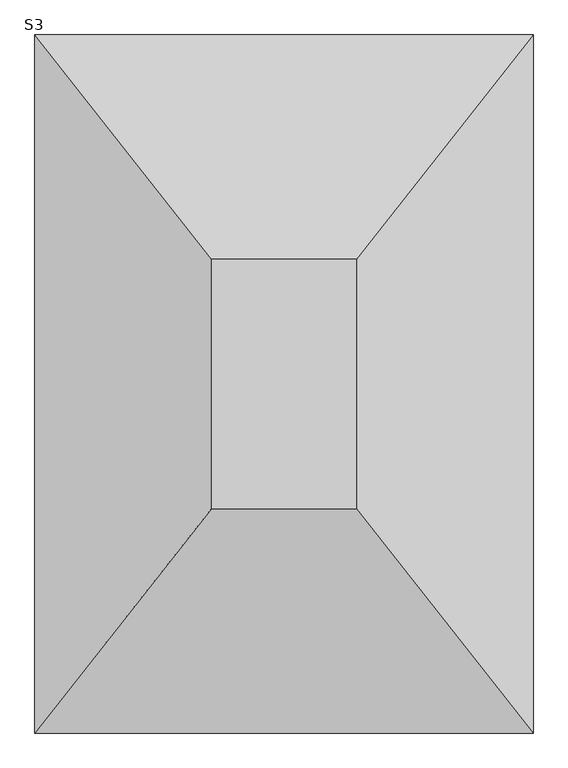
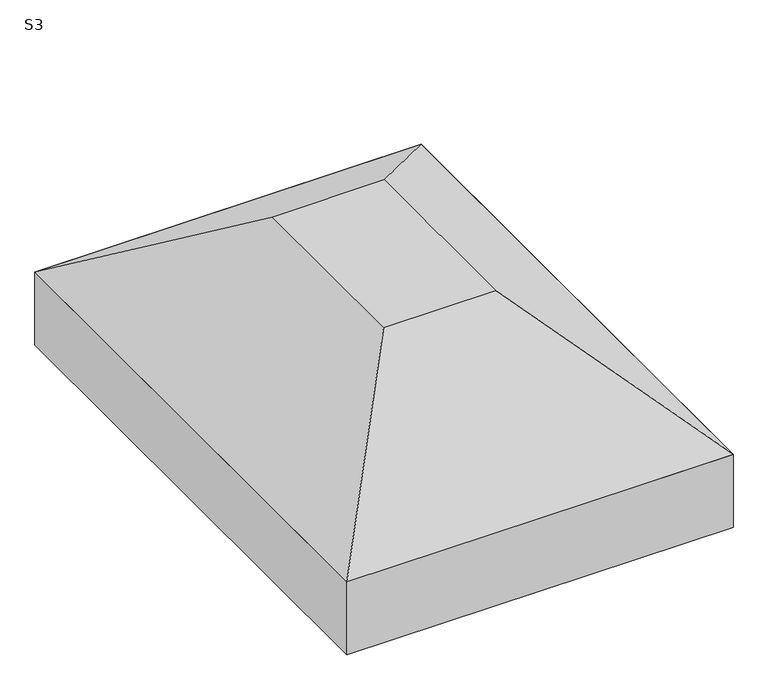
"""IFC4 building model written with IfcOpenShell, lengths in millimetres: fastener geometry, TQS - Sapata : S3."""

from ifc_helpers import new_model, si_unit, frame, origin, place, context, project, spatial, polyline, outline, extrude, faceted_brep, source, transform, mapped, element, save


def s3_fc183e28(model_context):
    return source(origin(), model_context, "Body", "SolidModel", [
        faceted_brep([(-55.0, 50.0, 0.0), (-345.0, 50.0, 0.0), (-345.0, -450.0, 0.0), (-55.0, -450.0, 0.0), (300.0, 500.0, -300.0), (300.0, -900.0, -300.0), (-700.0, -900.0, -300.0), (-700.0, 500.0, -300.0)], [[[0, 1, 2, 3]], [[4, 5, 6, 7]], [[4, 7, 1, 0]], [[7, 6, 2, 1]], [[6, 5, 3, 2]], [[5, 4, 0, 3]]]),
        extrude(outline(polyline([(300.0, 500.0), (300.0, -900.0), (-700.0, -900.0), (-700.0, 500.0), (300.0, 500.0)])), frame((0.0, 0.0, -500.0), z_axis=(0.0, 0.0, 1.0), x_axis=(1.0, 0.0, 0.0)), (0.0, 0.0, 1.0), 200.0),
    ])


if __name__ == "__main__":
    model = new_model("IFC4")
    model_context = context("Model", 3, world=origin())
    ifc_project = project(units=[si_unit("LENGTHUNIT", "METRE", prefix="MILLI")], contexts=[model_context])
    site = spatial("IfcSite", under=ifc_project)
    building = spatial("IfcBuilding", under=site)
    placement = place(None, origin())
    s3_shape = s3_fc183e28(model_context)
    element("IfcFastener", 1, ObjectType="TQS - Sapata : S3", at=placement, inside=building, context=model_context, shape_type="MappedRepresentation", body=[
        mapped(s3_shape, transform((0.0, 0.0, 0.0), x_axis=(1.0, 0.0, 0.0), y_axis=(0.0, 1.0, 0.0), z_axis=(0.0, 0.0, 1.0))),
    ])
    save(model, "model.ifc")

# Revit data of these elements
# Type "TQS - Sapata : S3"
#   TY = 0.50 m
#   TX = 0.29 m
#   HS = 0.50 m
#   H0 = 0.20 m
#   EXCYABS = 0.70 m
#   EXCY = 0.00 m
#   EXCXABS = 0.50 m
#   EXCX = 0.00 m
#   DIMY = 1.40 m
#   DIMX = 1.00 m
#   Material estrutural = Concreto - Concreto concretado no local
#   Width = 0
#   Length = 0
# Element 1 (IfcFastener, "TQS - Sapata : S3")
#   Materials on its faces: "Concreto - Concreto concretado no local"
# Materials
#   "Concreto - Concreto concretado no local": class "Concreto", colour RGB 192 192 192, transparency 0
